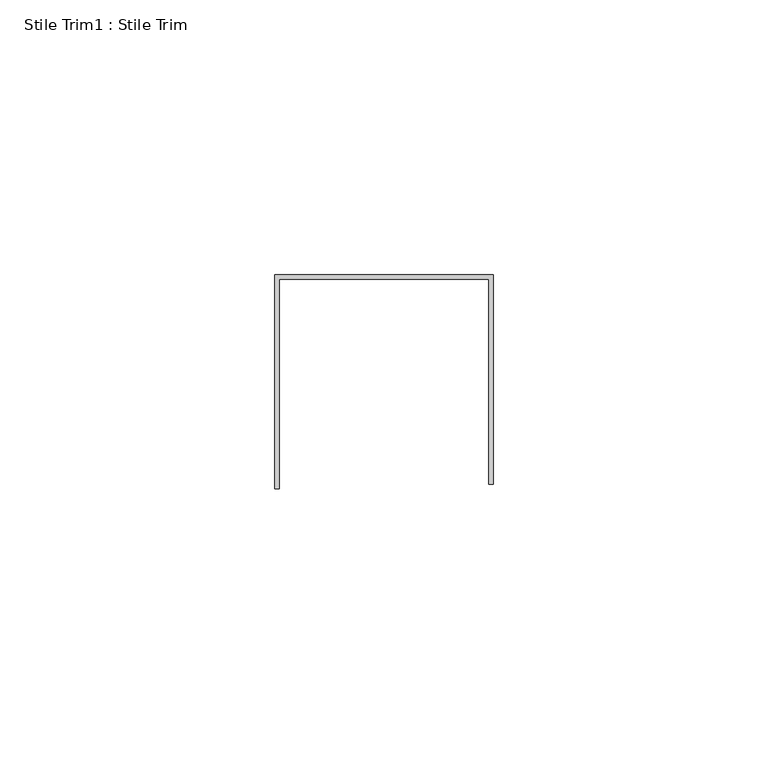
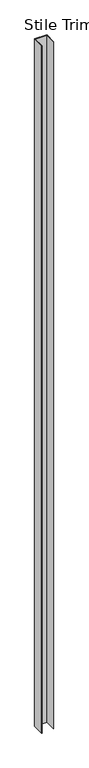
"""IFC4 building model written with IfcOpenShell, lengths in millimetres: proxy geometry, Stile Trim1 : Stile Trim."""

from ifc_helpers import new_model, si_unit, frame, origin, place, context, project, spatial, polyline, outline, extrude, source, transform, mapped, element, save


def stile_trim1_stile_trim_b98e89d7(model_context):
    return source(origin(), model_context, "Body", "SweptSolid", [
        extrude(outline(polyline([(587327.0060739, -532883.0289841), (587366.6808739, -532883.0289841), (587366.6808739, -532921.1289841), (587365.8934739, -532921.1289841), (587365.8934739, -532883.8163841), (587327.7934739, -532883.8163841), (587327.7934739, -532921.9163841), (587327.0060739, -532921.9163841), (587327.0060739, -532883.0289841)])), frame((0.0, 0.0, 50.8), z_axis=(0.0, 0.0, 1.0), x_axis=(1.0, 0.0, 0.0)), (0.0, 0.0, 1.0), 2350.3929688),
    ])


if __name__ == "__main__":
    model = new_model("IFC4")
    model_context = context("Model", 3, world=origin())
    ifc_project = project(units=[si_unit("LENGTHUNIT", "METRE", prefix="MILLI")], contexts=[model_context])
    site = spatial("IfcSite", under=ifc_project)
    building = spatial("IfcBuilding", under=site)
    placement = place(None, origin())
    stile_trim1_stile_trim_shape = stile_trim1_stile_trim_b98e89d7(model_context)
    element("IfcBuildingElementProxy", 1, Name="Stile Trim1 : Stile Trim", ObjectType="Stile Trim1 : Stile Trim", at=placement, inside=building, context=model_context, shape_type="MappedRepresentation", body=[
        mapped(stile_trim1_stile_trim_shape, transform((0.0, 0.0, 0.0), x_axis=(1.0, 0.0, 0.0), y_axis=(0.0, 1.0, 0.0), z_axis=(0.0, 0.0, 1.0))),
    ])
    save(model, "model.ifc")

# Revit data of these elements
# Element 1 (IfcBuildingElementProxy, "Stile Trim1 : Stile Trim")
#   Materials on its faces: "EDGE TRIM BY MTL PANEL MFR."
# Materials
#   "EDGE TRIM BY MTL PANEL MFR.": class "Generic", colour RGB 239 242 240, transparency 0, Cost = 0
